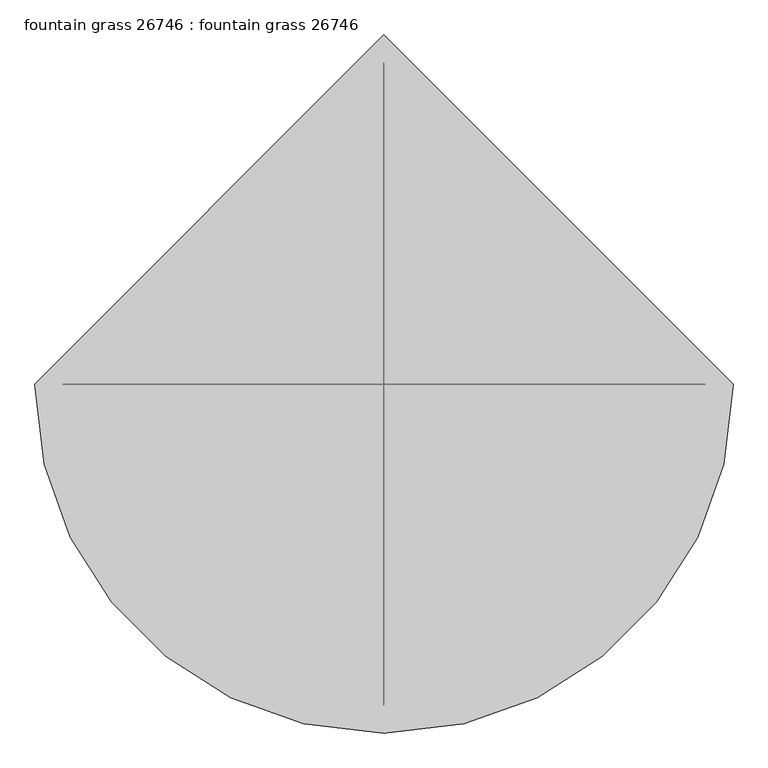
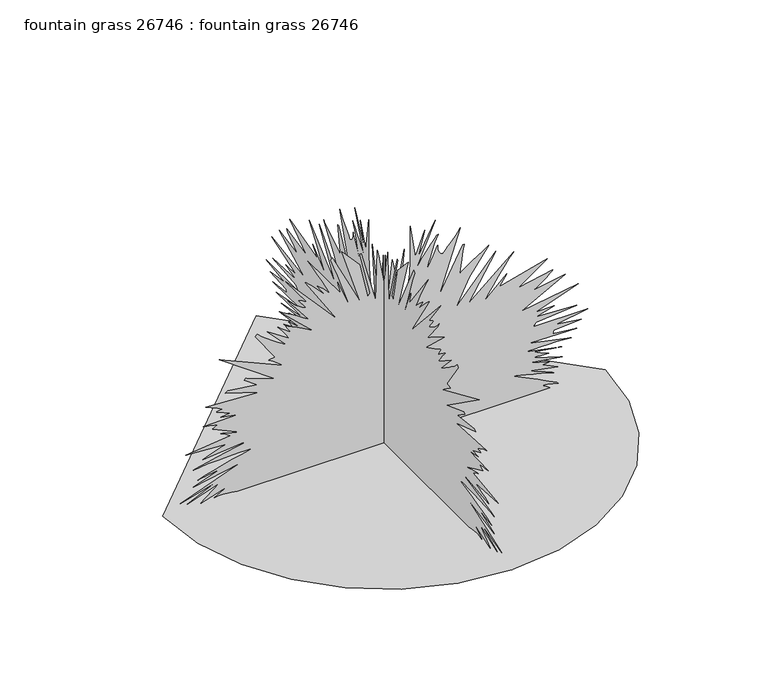
"""IFC4 building model written with IfcOpenShell, lengths in millimetres: proxy geometry, fountain grass 26746 : fountain grass 26746."""

from ifc_helpers import new_model, si_unit, origin, place, context, project, spatial, triangles, source, transform, mapped, element, save


def fountain_grass_26746_fountain_grass_26746_31a79539(model_context):
    return source(origin(), model_context, "Body", "Tessellation", [
        triangles([(-1075.1021822, 0.0, 0.0), (-1046.6796438, -246.3421583, 0.0), (-965.7324045, -472.5690837, 0.0), (-838.7452429, -672.1950891, 0.0), (-672.1950891, -838.7452429, 0.0), (-472.5690837, -965.7324045, 0.0), (-246.341904, -1046.6796438, 0.0), (4.7e-05, -1075.1021822, 0.0), (246.3421583, -1046.6796438, 0.0), (472.5690837, -965.7324045, 0.0), (672.1950891, -838.7452429, 0.0), (838.7452429, -672.1950891, 0.0), (965.7324045, -472.5690837, 0.0), (1046.6796438, -246.341904, 0.0), (1075.1021822, 9.4e-05, 0.0), (-0.000141, 1075.1021822, 0.0), (-0.0002094, 151.7493584, 903.5253731), (-0.0002064, 197.8505688, 1023.5783649), (-0.0002098, 163.2745906, 893.9190554), (-0.000206, 247.7932689, 1057.1952084), (-0.0002115, 151.7493584, 831.4910345), (-0.0002109, 167.7051159, 857.3634378), (-0.0002104, 186.8993659, 885.4837418), (-0.0002098, 207.3806375, 913.5837708), (-0.0002093, 227.1984504, 939.3926605), (-0.0002089, 244.4013429, 960.6372213), (-0.0002086, 257.0401245, 975.0516758), (-0.0002085, 263.1615169, 980.3602907), (-0.0002094, 247.7267213, 943.5176268), (-0.0002103, 234.4486256, 908.2090988), (-0.0002111, 223.4664289, 876.1391087), (-0.0002118, 214.9206206, 848.9967247), (-0.0002123, 208.9511085, 828.4836599), (-0.0002127, 205.6989088, 816.294215), (-0.0002127, 205.3039292, 814.1250887), (-0.0002127, 208.3029104, 818.0239786), (-0.0002124, 216.0537091, 832.5501995), (-0.000212, 226.6881618, 853.6500017), (-0.0002116, 238.3378685, 877.271961), (-0.0002112, 249.1338665, 899.3648712), (-0.0002109, 257.207756, 915.8748373), (-0.0002107, 260.692645, 922.748037), (-0.0002103, 260.2582965, 906.3549242), (-0.0002103, 263.0522939, 893.568568), (-0.0002106, 267.949415, 883.9953152), (-0.0002111, 273.8345936, 877.2388962), (-0.0002116, 279.5876763, 872.9031143), (-0.000212, 284.0860209, 870.5917728), (-0.0002121, 286.2119994, 869.908457), (-0.0002118, 297.8807457, 886.1644415), (-0.0002115, 309.7933362, 900.0811066), (-0.0002113, 321.8837319, 912.8293837), (-0.0002111, 334.0884012, 925.5801315), (-0.0002109, 346.3388163, 939.504427), (-0.0002105, 358.5765141, 955.7731287), (-0.0002101, 370.7304234, 975.5571682), (-0.0002182, 267.0019983, 658.6111799), (-0.000213, 382.2543929, 884.3153538), (-0.0002131, 389.9378629, 884.3153538), (-0.0002137, 385.7570498, 861.6865025), (-0.0002144, 381.2002785, 835.410272), (-0.0002152, 376.6689054, 808.0824343), (-0.0002159, 372.5719171, 782.3039932), (-0.0002165, 369.305474, 760.6733368), (-0.0002169, 367.2760194, 745.7889982), (-0.0002171, 366.8873803, 740.2492201), (-0.0002169, 377.1819918, 749.4998909), (-0.0002168, 398.429096, 764.5798571), (-0.0002166, 426.0591682, 782.8856438), (-0.0002164, 455.5053723, 801.8137035), (-0.0002163, 482.19564, 818.763105), (-0.0002161, 501.5631351, 831.122743), (-0.0002161, 509.0332824, 836.294157), (-0.0002187, 412.9883454, 706.6349201), (-0.0002218, 347.6799408, 572.1725244), (-0.0002178, 543.6077345, 793.0735394), (-0.0002226, 409.1478822, 572.1725244), (-0.0002221, 630.0006443, 760.9578398), (-0.0002225, 607.1482965, 733.4877869), (-0.0002229, 581.7076618, 698.9640947), (-0.0002232, 555.6879564, 661.3112331), (-0.0002235, 531.0982146, 624.4456781), (-0.0002238, 509.9451453, 592.2867763), (-0.000224, 494.2377829, 568.7536923), (-0.0002241, 485.9827998, 557.7656639), (-0.0002226, 597.394713, 658.6111799), (-0.0002236, 558.9747108, 605.7868607), (-0.0002249, 793.3225067, 668.217425), (-0.000226, 651.1791481, 567.3694018), (-0.0002272, 820.215996, 600.9862453), (-0.0002273, 814.2901949, 595.3652584), (-0.0002274, 803.8635057, 586.2314046), (-0.0002276, 790.0737951, 574.7607748), (-0.0002278, 774.0693214, 562.1243005), (-0.0002279, 756.9878059, 549.4928767), (-0.000228, 739.9748909, 538.045138), (-0.0002281, 724.171059, 528.951943), (-0.0002293, 881.683901, 557.7656639), (-0.0002299, 666.5461607, 442.5132874), (-0.0002323, 943.1518787, 485.7338688), (-0.0002317, 735.6975357, 413.6995302), (-0.0002329, 827.8994659, 413.6995302), (-0.0002325, 739.5380716, 389.6889682), (-0.0002353, 935.4683361, 380.0852303), (-0.0002333, 739.5380716, 360.875211), (-0.0002334, 737.0615513, 358.3860097), (-0.0002334, 734.2345436, 355.2567312), (-0.0002335, 731.3236748, 351.8201314), (-0.0002335, 728.5931728, 348.4089297), (-0.0002336, 726.3148235, 345.3558457), (-0.0002336, 724.7527096, 342.9987222), (-0.0002337, 724.171059, 341.6677714), (-0.0002372, 989.2528439, 341.6677714), (-0.0002359, 835.5829359, 317.6571731), (-0.0002381, 958.5188187, 298.4471538), (-0.0002366, 824.0564592, 288.843434), (-0.000237, 820.215996, 274.4365736), (-0.0002389, 935.4683361, 260.0296949), (-0.0002357, 704.9635832, 264.8328356), (-0.0002397, 908.5748468, 221.6119818), (-0.0002392, 879.3065025, 224.4689658), (-0.0002387, 841.8263048, 226.3310433), (-0.0002381, 800.7671831, 227.3607588), (-0.0002376, 760.7622849, 227.7214381), (-0.0002371, 726.4494083, 227.5753896), (-0.0002368, 702.461701, 227.0854304), (-0.0002367, 693.4371065, 226.4143594), (-0.0002399, 862.4738817, 192.7990239), (-0.0002375, 720.3305958, 212.0077533), (-0.0002395, 801.079664, 180.0418811), (-0.0002393, 789.8198135, 180.8544223), (-0.0002391, 775.0700598, 181.8744909), (-0.0002389, 758.976638, 182.9049694), (-0.0002386, 743.6934866, 183.7490131), (-0.0002385, 731.3642973, 184.2100133), (-0.0002384, 724.1406103, 184.090889), (-0.0002384, 724.171059, 183.194523), (-0.0002416, 866.3169611, 139.9746865), (-0.0002388, 708.8040464, 163.9857935), (-0.0002409, 802.8830423, 135.5523002), (-0.0002408, 799.4514931, 134.831959), (-0.0002408, 794.1606823, 134.0915427), (-0.0002407, 787.8817778, 133.3391994), (-0.0002407, 781.4835491, 132.5827867), (-0.0002406, 775.8346207, 131.8306978), (-0.0002406, 771.8087036, 131.0902815), (-0.0002406, 770.2720242, 130.3701946), (-0.0002426, 843.2664785, 96.75485), (-0.0002398, 697.2953739, 122.86552), (-0.0002401, 707.9455233, 119.2147799), (-0.0002406, 727.4654074, 112.0362392), (-0.0002412, 752.0246641, 102.744419), (-0.0002418, 777.7954748, 92.7543584), (-0.0002424, 800.9424631, 83.4810781), (-0.0002428, 817.6404264, 76.3393719), (-0.000243, 824.0564592, 72.7440018), (-0.0002423, 793.2310152, 81.617738), (-0.0002416, 757.9402914, 91.2158803), (-0.0002408, 721.5396063, 100.7012479), (-0.0002401, 687.3868217, 109.2361467), (-0.0002395, 658.8372562, 115.9836545), (-0.0002392, 639.2462282, 120.1060682), (-0.000239, 631.9691288, 120.7659571), (-0.00024, 666.4089598, 103.8820858), (-0.0002411, 705.799288, 84.5753155), (-0.0002422, 746.4087278, 64.5205076), (-0.0002433, 784.498554, 45.3925509), (-0.0002442, 816.3297506, 28.8660546), (-0.0002449, 838.1686792, 16.6156986), (-0.0002452, 846.2788673, 10.3164533), (-0.0002449, 834.4653442, 14.1385651), (-0.0002446, 820.7849293, 17.3725156), (-0.0002444, 806.5482256, 20.018432), (-0.0002441, 793.0684525, 22.0761847), (-0.0002439, 781.6562857, 23.5461577), (-0.0002438, 773.6197123, 24.4280193), (-0.0002437, 770.2720242, 24.7219217), (-0.0002438, 772.6468792, 22.8719915), (-0.000244, 777.9732983, 19.2397436), (-0.0002442, 785.103023, 14.5784422), (-0.0002445, 792.8881582, 9.6414491), (-0.0002447, 800.1804457, 5.1824076), (-0.0002449, 805.8319902, 1.9544036), (-0.000245, 808.6894466, 0.7109504), (-0.0002248, -712.2762182, 7.55e-05), (-0.0002247, -716.251339, 1.888295), (-0.0002245, -727.0437761, 4.4398649), (-0.0002242, -742.9644613, 7.0367071), (-0.0002239, -762.3193119, 9.0605264), (-0.0002236, -783.416498, 9.8934675), (-0.0002233, -804.5594662, 8.9170168), (-0.0002232, -824.0564592, 5.5131917), (-0.0002229, -758.7480183, 43.9307805), (-0.0002224, -893.2079069, 0.7110012), (-0.0002215, -801.0059767, 72.7440018), (-0.000221, -954.6783554, 19.9198029), (-0.000221, -820.215996, 82.3482439), (-0.0002201, -989.2528439, 34.3262887), (-0.0002208, -701.1205765, 139.9746865), (-0.0002191, -927.7848661, 96.75485), (-0.0002194, -808.6894466, 139.9746865), (-0.0002193, -812.3292681, 139.9878942), (-0.0002192, -822.1235104, 138.9035673), (-0.0002191, -836.3982931, 136.9663127), (-0.000219, -853.4747217, 134.4199656), (-0.0002188, -871.6762997, 131.5086244), (-0.0002187, -889.3216616, 128.4766238), (-0.0002185, -904.7343836, 125.5680804), (-0.0002186, -893.5940025, 129.4418265), (-0.0002187, -867.1881289, 137.4656826), (-0.0002189, -829.5479118, 148.2962261), (-0.0002191, -784.7068262, 160.5885445), (-0.0002194, -736.7034336, 172.9992332), (-0.0002196, -689.5686653, 184.1843608), (-0.0002199, -647.3361414, 192.7990239), (-0.0002198, -647.3361414, 197.6011291), (-0.0002195, -670.2748575, 197.8660475), (-0.000219, -707.9862185, 197.3700022), (-0.0002184, -755.0320387, 196.1048178), (-0.0002178, -805.9742054, 194.0624097), (-0.0002172, -855.3746058, 191.2351477), (-0.0002168, -897.79004, 187.6151289), (-0.0002165, -927.7848661, 183.194523), (-0.0002165, -918.4681383, 186.3568118), (-0.0002167, -893.3831142, 192.5249491), (-0.0002169, -856.8325836, 200.7720656), (-0.0002172, -813.1090897, 210.171837), (-0.0002176, -766.5153494, 219.7974123), (-0.0002179, -721.3516817, 228.7219402), (-0.0002182, -681.9131006, 236.0185879), (-0.0002181, -681.9131006, 240.8209655), (-0.000216, -881.683901, 221.6119818), (-0.000216, -877.2592438, 223.6533724), (-0.000216, -864.5567488, 228.9396232), (-0.000216, -846.1366522, 236.2129074), (-0.0002161, -824.5568647, 244.2159255), (-0.0002161, -802.3750065, 251.6913958), (-0.0002162, -782.1465174, 257.3830178), (-0.0002164, -766.4315609, 260.0296949), (-0.0002133, -962.3618254, 274.4365736), (-0.0002155, -747.2215416, 298.4471538), (-0.0002154, -748.9690367, 300.212453), (-0.0002152, -753.6680231, 303.7532252), (-0.000215, -760.5209478, 308.3607565), (-0.0002147, -768.7124537, 313.3315287), (-0.0002145, -777.4449875, 317.9594075), (-0.0002143, -785.9107498, 321.5357517), (-0.0002141, -793.3021591, 323.3569342), (-0.0002142, -787.9021254, 322.9682951), (-0.0002145, -773.9448378, 319.7958507), (-0.0002149, -754.7907017, 314.8758748), (-0.0002153, -733.8001951, 309.2421344), (-0.0002157, -714.3387377, 303.9360992), (-0.0002161, -699.7641912, 299.9914817), (-0.0002162, -693.4371065, 298.4471538), (-0.0002125, -831.7399292, 360.875211), (-0.0002125, -830.7239302, 362.5795401), (-0.0002124, -827.9833271, 364.8223901), (-0.0002124, -823.9904022, 367.3496704), (-0.0002124, -819.2127142, 369.9125227), (-0.0002124, -814.1174583, 372.2544219), (-0.0002124, -809.1745914, 374.1289078), (-0.0002124, -804.8489834, 375.2820714), (-0.0002124, -807.681078, 376.3869822), (-0.0002122, -815.2883898, 378.2437366), (-0.000212, -826.3196205, 380.5906863), (-0.0002117, -839.4361164, 383.168763), (-0.0002115, -853.2892679, 385.7163909), (-0.0002112, -866.5404213, 387.9770087), (-0.000211, -877.8408943, 389.6889682), (-0.0002131, -712.6470531, 394.4920907), (-0.0002116, -793.3225067, 408.8989511), (-0.0002121, -743.3810783, 413.6995302), (-0.0002103, -812.5324533, 442.5132874), (-0.0002103, -811.3640654, 443.8569191), (-0.0002103, -808.2246494, 445.132023), (-0.0002103, -803.6476032, 446.2470712), (-0.0002104, -798.178969, 447.1106812), (-0.0002104, -792.3547606, 447.6364486), (-0.0002105, -786.7133898, 447.7354978), (-0.0002106, -781.7985008, 447.31641), (-0.0002105, -785.3392731, 449.5770278), (-0.0002102, -794.7525066, 454.4588882), (-0.0002098, -808.222106, 461.0349403), (-0.0002094, -823.9294321, 468.375517), (-0.000209, -840.0584621, 475.5561107), (-0.0002086, -854.7929552, 481.6521049), (-0.0002083, -866.3169611, 485.7338688), (-0.0002122, -605.078183, 471.3270083), (-0.0002084, -770.2720242, 524.1513276), (-0.0002083, -758.7480183, 533.7550655), (-0.0002108, -616.6021889, 514.5450826), (-0.0002087, -678.0700939, 557.7656639), (-0.0002085, -670.386624, 567.3694018), (-0.0002119, -528.2407219, 514.5450826), (-0.0002026, -801.0059767, 706.6349201), (-0.0002107, -493.6662698, 572.1725244), (-0.0002103, -502.7518707, 579.84077), (-0.0002099, -513.8160936, 588.6494983), (-0.0002095, -525.7210719, 597.7502872), (-0.0002091, -537.32883, 606.3024905), (-0.0002087, -547.4989941, 613.4576134), (-0.0002085, -555.0935886, 618.3700315), (-0.0002084, -558.9772542, 620.1936848), (-0.0002084, -557.3414892, 621.3672323), (-0.0002084, -553.1149303, 622.2358566), (-0.0002085, -547.2958088, 622.8886511), (-0.0002085, -540.8924569, 623.4067881), (-0.0002086, -534.9133161, 623.8742014), (-0.0002086, -530.3616317, 624.3770777), (-0.0002086, -528.2407219, 624.99688), (-0.0002032, -624.2856588, 764.2598185), (-0.000203, -616.6021889, 773.8661362), (-0.0002039, -593.2849711, 753.716276), (-0.0002049, -567.5725871, 733.8154558), (-0.0002058, -541.6163589, 715.1616526), (-0.0002066, -517.5625946, 698.7558226), (-0.0002072, -497.5601091, 685.596088), (-0.0002077, -483.7552105, 676.68326), (-0.0002079, -478.2992935, 673.0180767), (-0.0002038, -566.6607242, 769.062941), (-0.0002074, -459.0893106, 697.0286751), (-0.0002072, -461.8096387, 701.9384771), (-0.0002069, -466.5873631, 709.5711508), (-0.0002066, -473.2904423, 719.5050648), (-0.0002061, -481.786726, 731.3211313), (-0.0002056, -491.9467163, 744.6002626), (-0.000205, -503.6332486, 758.9207548), (-0.0002044, -516.7167523, 773.8661362), (-0.0002045, -513.2318996, 772.2836746), (-0.0002048, -504.2098123, 766.0124004), (-0.0002052, -491.8044648, 756.8075117), (-0.0002057, -478.1697593, 746.4290754), (-0.0002062, -465.4570905, 736.6373766), (-0.0002065, -455.8177806, 729.1875406), (-0.0002067, -451.4058043, 725.842396), (-0.0002064, -455.2462675, 731.5675552), (-0.0002062, -459.8665524, 738.7150841), (-0.0002059, -464.8017526, 746.5230377), (-0.0002056, -469.5794769, 754.2243118), (-0.0002053, -473.7349282, 761.0594324), (-0.0002051, -476.7956062, 766.2588243), (-0.000205, -478.2992935, 769.062941), (-0.0002053, -467.4382559, 763.1752916), (-0.0002059, -448.0021966, 753.3581583), (-0.0002066, -423.3616948, 740.947724), (-0.0002073, -396.8746124, 727.2876566), (-0.0002081, -371.9089851, 713.7214788), (-0.0002087, -351.8277617, 701.5879171), (-0.0002091, -339.9964345, 692.2280233), (-0.0002022, -509.0332824, 850.7010538), (-0.0002024, -501.3497761, 846.621797), (-0.000203, -481.4362023, 834.9479456), (-0.0002039, -453.9940547, 818.4430664), (-0.0002048, -423.7299863, 799.8731243), (-0.0002057, -395.3480704, 782.0093164), (-0.0002064, -373.5523441, 767.6151369), (-0.0002068, -363.0469171, 759.4592394), (-0.0002065, -368.546, 766.7414257), (-0.0002058, -383.526917, 785.5628059), (-0.0002047, -404.1618493, 811.3869564), (-0.0002036, -426.6281379, 839.67491), (-0.0002025, -447.1030509, 865.8851561), (-0.0002018, -461.7588424, 885.4786549), (-0.0002014, -466.7727805, 893.9190554), (-0.0002023, -448.2638449, 874.4677717), (-0.000203, -430.4813184, 858.5800787), (-0.0002036, -414.1669072, 846.0858559), (-0.000204, -400.0597741, 836.8173809), (-0.0002044, -388.9066395, 830.6070768), (-0.0002046, -381.4441226, 827.2873667), (-0.0002046, -378.4138933, 826.687912), (-0.0002027, -412.9883454, 874.7116522), (-0.0002028, -410.1994168, 874.6379648), (-0.0002029, -404.7105077, 872.2808413), (-0.0002031, -397.603565, 868.4733702), (-0.0002034, -389.9581741, 864.0537998), (-0.0002036, -382.8487244, 859.8627766), (-0.0002037, -377.3623587, 856.730991), (-0.0002038, -374.5708866, 855.5016329), (-0.0001983, -478.2992935, 994.7671148), (-0.0002099, -228.5847938, 716.2386217), (-0.0002007, -382.2543929, 956.3471489), (-0.0002008, -377.5401458, 953.682704), (-0.0002013, -366.727361, 944.1653343), (-0.0002019, -351.5610629, 929.5552523), (-0.0002027, -333.7912173, 911.6203005), (-0.0002035, -315.1705153, 892.1258509), (-0.0002043, -297.4463973, 872.8294996), (-0.000205, -282.3689745, 855.5016329), (-0.0002026, -324.6294582, 917.9296537), (-0.0002027, -320.6416566, 916.0831095), (-0.000203, -312.1021706, 909.1260487), (-0.0002035, -300.8906456, 898.981319), (-0.000204, -288.8891434, 887.5817968), (-0.0002045, -277.9849398, 876.8528732), (-0.0002048, -270.0626945, 868.7172506), (-0.000205, -267.0019983, 865.1053345), (-0.0002046, -271.2920526, 874.9732641), (-0.0002037, -283.4510124, 899.7559811), (-0.0002024, -300.8601605, 934.157733), (-0.000201, -320.9083554, 972.880006), (-0.0001996, -340.9768616, 1010.6243591), (-0.0001985, -358.4571536, 1042.097438), (-0.0001977, -370.7304234, 1061.9957874), (-0.0002064, -209.3757919, 841.0947361), (-0.0002061, -212.3376932, 849.9161453), (-0.0002058, -215.4885547, 860.5994322), (-0.0002054, -218.5616956, 872.0446638), (-0.000205, -221.2901628, 883.1571396), (-0.0002047, -223.4082747, 892.8396154), (-0.0002045, -224.6477885, 899.9947746), (-0.0002044, -224.7430407, 903.5253731), (-0.0002098, -163.2748449, 749.8529943), (-0.0002094, -166.4719427, 760.9984623), (-0.0002084, -175.9733068, 790.7926466), (-0.0002069, -190.101278, 833.7744707), (-0.0002052, -207.1779428, 884.4830034), (-0.0002033, -225.5248425, 937.4622551), (-0.0002016, -243.4645905, 987.2487511), (-0.0002002, -259.318492, 1028.3814875), (-0.0002, -251.6352582, 1037.9851891), (-0.0002099, -116.1998023, 765.6542828), (-0.0002002, -205.5340569, 1052.3920858), (-0.0002042, -117.1738889, 956.3471489), (-0.00021, -78.7561757, 778.6667152), (-0.00021, -77.3934682, 780.4573763), (-0.0002099, -75.5994689, 782.9009045), (-0.0002099, -73.577631, 785.6593117), (-0.0002098, -71.5275972, 788.3949005), (-0.0002098, -69.6525708, 790.7697556), (-0.0002097, -68.1529576, 792.4410925), (-0.0002097, -67.2306846, 793.0735394), (-0.0002026, -117.1738889, 1009.1714682), (-0.0002027, -109.4901464, 1009.1714682), (-0.0002115, -40.3384626, 745.0523426), (-0.000204, -32.6549699, 999.5677666), (-0.0002043, -30.2686421, 991.1984373), (-0.0002051, -25.7212838, 968.6636209), (-0.0002061, -19.6890689, 935.823983), (-0.0002074, -12.8482471, 896.5454212), (-0.0002087, -5.8757252, 854.6837322), (-0.00021, 0.5533969, 814.1047411), (-0.0002111, 5.7626445, 778.6667152), (-0.0002057, 5.7626445, 961.1502714), (-0.0002127, 17.2877302, 730.6455185), (-0.0002072, 40.3384626, 927.5359715), (-0.0002115, 67.2306846, 793.0735394), (-0.0002069, 97.9646508, 961.1502714), (-0.0002145, 74.9141773, 697.0286751), (-0.0002143, 99.6672177, 714.3946209), (-0.0002131, 115.3773507, 759.9418407), (-0.0002114, 124.0562722, 823.853274), (-0.0002092, 127.7161506, 896.3143307), (-0.0002071, 128.3684273, 967.5027906), (-0.0002053, 128.0255249, 1027.6042093), (-0.0002042, 128.6986215, 1066.79891), (151.7493584, -7.84e-05, 903.5253731), (197.8503144, -8.55e-05, 1023.5783649), (163.2745906, -7.78e-05, 893.9190554), (247.7932689, -8.75e-05, 1057.1952084), (151.7493584, -7.41e-05, 831.4910345), (167.7048616, -7.56e-05, 857.3634378), (186.8991115, -7.73e-05, 885.4837418), (207.3803832, -7.9e-05, 913.5837708), (227.1984504, -8.05e-05, 939.3901171), (244.4013429, -8.18e-05, 960.6372213), (257.0401245, -8.26e-05, 975.0516758), (263.1615169, -8.29e-05, 980.3602907), (247.726467, -8.07e-05, 943.5176268), (234.4483712, -7.86e-05, 908.2090988), (223.4661746, -7.67e-05, 876.1391087), (214.9203662, -7.51e-05, 848.9967247), (208.9508542, -7.39e-05, 828.4811165), (205.6986544, -7.32e-05, 816.294215), (205.3036749, -7.3e-05, 814.1250887), (208.3026561, -7.32e-05, 818.0239786), (216.0534548, -7.4e-05, 832.5501995), (226.6879074, -7.52e-05, 853.6500017), (238.3376142, -7.65e-05, 877.271961), (249.1336122, -7.77e-05, 899.3623278), (257.207756, -7.86e-05, 915.8748373), (260.692645, -7.9e-05, 922.748037), (260.2582965, -7.89e-05, 906.3549242), (263.0522939, -7.86e-05, 893.568568), (267.949415, -7.8e-05, 883.9953152), (273.8345936, -7.75e-05, 877.2388962), (279.5876763, -7.69e-05, 872.9031143), (284.0860209, -7.65e-05, 870.5917728), (286.2119994, -7.64e-05, 869.908457), (297.8807457, -7.73e-05, 886.1644415), (309.7933362, -7.82e-05, 900.0811066), (321.8837319, -7.89e-05, 912.8293837), (334.0884012, -7.97e-05, 925.5801315), (346.3388163, -8.05e-05, 939.504427), (358.5765141, -8.15e-05, 955.7731287), (370.7304234, -8.27e-05, 975.5571682), (267.0019983, -6.38e-05, 658.6111799), (382.2543929, -7.72e-05, 884.3153538), (389.9378629, -7.72e-05, 884.3153538), (385.7570498, -7.59e-05, 861.6865025), (381.2002785, -7.43e-05, 835.410272), (376.6689054, -7.27e-05, 808.0824343), (372.5693736, -7.11e-05, 782.3039932), (369.305474, -6.98e-05, 760.6733368), (367.2760194, -6.9e-05, 745.7889982), (366.8873803, -6.86e-05, 740.2492201), (377.1819918, -6.92e-05, 749.4998909), (398.429096, -7.01e-05, 764.5798571), (426.0591682, -7.12e-05, 782.8856438), (455.5053723, -7.23e-05, 801.8137035), (482.19564, -7.33e-05, 818.763105), (501.5631351, -7.4e-05, 831.122743), (509.0332824, -7.43e-05, 836.294157), (412.9883454, -6.66e-05, 706.6349201), (347.6799408, -5.86e-05, 572.1725244), (543.6077345, -7.18e-05, 793.0735394), (409.1478822, -5.86e-05, 572.1725244), (629.9981009, -6.77e-05, 760.9578398), (607.145753, -6.62e-05, 733.4877869), (581.7076618, -6.44e-05, 698.9640947), (555.6879564, -6.26e-05, 661.3112331), (531.0982146, -6.09e-05, 624.4456781), (509.9451453, -5.94e-05, 592.2867763), (494.2377829, -5.83e-05, 568.7536923), (485.9827998, -5.77e-05, 557.7656639), (597.3921696, -6.38e-05, 658.6111799), (558.9747108, -6.06e-05, 605.7868607), (793.3225067, -6.43e-05, 668.217425), (651.1791481, -5.83e-05, 567.3694018), (820.215996, -6.03e-05, 600.9862453), (814.2901949, -6e-05, 595.3652584), (803.8635057, -5.94e-05, 586.2314046), (790.0737951, -5.88e-05, 574.7607748), (774.0693214, -5.8e-05, 562.1243005), (756.9878059, -5.73e-05, 549.4928767), (739.9748909, -5.66e-05, 538.045138), (724.171059, -5.6e-05, 528.951943), (881.683901, -5.77e-05, 557.7656639), (666.5461607, -5.09e-05, 442.5132874), (943.1518787, -5.35e-05, 485.7338688), (735.6975357, -4.92e-05, 413.6995302), (827.8994659, -4.92e-05, 413.6995302), (739.5380716, -4.77e-05, 389.6889682), (935.4683361, -4.72e-05, 380.0852303), (739.5380716, -4.6e-05, 360.875211), (737.0615513, -4.59e-05, 358.3860097), (734.2345436, -4.57e-05, 355.2567312), (731.3236748, -4.55e-05, 351.8201314), (728.5931728, -4.53e-05, 348.4089297), (726.3148235, -4.51e-05, 345.3558457), (724.7527096, -4.49e-05, 342.9987222), (724.171059, -4.49e-05, 341.6677714), (989.2528439, -4.49e-05, 341.6677714), (835.5829359, -4.34e-05, 317.6571731), (958.5188187, -4.23e-05, 298.4471538), (824.0564592, -4.17e-05, 288.843434), (820.215996, -4.09e-05, 274.4365736), (935.4683361, -4e-05, 260.0296949), (704.9635832, -4.03e-05, 264.8328356), (908.5748468, -3.77e-05, 221.6119818), (879.3065025, -3.79e-05, 224.4689658), (841.8263048, -3.8e-05, 226.3310433), (800.7647123, -3.81e-05, 227.3607588), (760.7622849, -3.81e-05, 227.7211837), (726.4494083, -3.81e-05, 227.5753896), (702.461701, -3.8e-05, 227.0854304), (693.4371065, -3.8e-05, 226.4141051), (862.4738817, -3.6e-05, 192.7987696), (720.3305958, -3.71e-05, 212.007499), (801.079664, -3.52e-05, 180.0418811), (789.8198135, -3.53e-05, 180.8544223), (775.0700598, -3.53e-05, 181.8744909), (758.976638, -3.54e-05, 182.9049694), (743.6934866, -3.55e-05, 183.7490131), (731.3642973, -3.55e-05, 184.2100133), (724.1406103, -3.55e-05, 184.090889), (724.171059, -3.54e-05, 183.194523), (866.3169611, -3.28e-05, 139.9746865), (708.8040464, -3.43e-05, 163.9857935), (802.8830423, -3.26e-05, 135.5523002), (799.4514931, -3.25e-05, 134.831959), (794.1606823, -3.25e-05, 134.0915427), (787.8817778, -3.24e-05, 133.3391994), (781.4810057, -3.24e-05, 132.5827867), (775.8346207, -3.24e-05, 131.8306978), (771.8087036, -3.23e-05, 131.0902815), (770.2720242, -3.23e-05, 130.3701946), (843.2664785, -3.03e-05, 96.75485), (697.2953739, -3.18e-05, 122.8652657), (707.9455233, -3.16e-05, 119.2147799), (727.4654074, -3.12e-05, 112.0362392), (752.0246641, -3.06e-05, 102.744419), (777.7954748, -3e-05, 92.7543584), (800.9424631, -2.95e-05, 83.4810781), (817.6404264, -2.91e-05, 76.3393719), (824.0564592, -2.88e-05, 72.7440018), (793.2310152, -2.94e-05, 81.617738), (757.9402914, -2.99e-05, 91.2158803), (721.5396063, -3.05e-05, 100.7012479), (687.3868217, -3.1e-05, 109.2361467), (658.8372562, -3.14e-05, 115.9836545), (639.2462282, -3.17e-05, 120.1060682), (631.9691288, -3.17e-05, 120.7659571), (666.4089598, -3.07e-05, 103.8820858), (705.799288, -2.95e-05, 84.5753155), (746.4087278, -2.83e-05, 64.5205076), (784.498554, -2.72e-05, 45.3925509), (816.3297506, -2.62e-05, 28.8660546), (838.1686792, -2.55e-05, 16.6156986), (846.2788673, -2.51e-05, 10.3164533), (834.4653442, -2.53e-05, 14.1385651), (820.7849293, -2.55e-05, 17.3724907), (806.5482256, -2.57e-05, 20.018432), (793.0684525, -2.58e-05, 22.0761598), (781.6562857, -2.59e-05, 23.5461577), (773.6197123, -2.6e-05, 24.4280193), (770.2720242, -2.6e-05, 24.7219217), (772.6468792, -2.59e-05, 22.8719915), (777.9732983, -2.56e-05, 19.2397436), (785.103023, -2.54e-05, 14.5784422), (792.8881582, -2.51e-05, 9.6414491), (800.1804457, -2.48e-05, 5.1824076), (805.8319902, -2.46e-05, 1.9544036), (808.6894466, -2.45e-05, 0.7109504), (-712.2762182, -2.45e-05, 3.05e-05), (-716.251339, -2.46e-05, 1.8882493), (-727.0437761, -2.48e-05, 4.4398141), (-742.9644613, -2.49e-05, 7.0366566), (-762.3193119, -2.5e-05, 9.0604759), (-783.416498, -2.51e-05, 9.8934175), (-804.5594662, -2.5e-05, 8.9169657), (-824.0564592, -2.48e-05, 5.5131406), (-758.7480183, -2.71e-05, 43.9307805), (-893.2104504, -2.45e-05, 0.7109504), (-801.0059767, -2.88e-05, 72.7440018), (-954.6783554, -2.57e-05, 19.919753), (-820.215996, -2.94e-05, 82.3482439), (-989.2528439, -2.65e-05, 34.3262887), (-701.1205765, -3.28e-05, 139.9746865), (-927.7848661, -3.03e-05, 96.75485), (-808.6894466, -3.28e-05, 139.9746865), (-812.3292681, -3.28e-05, 139.9878942), (-822.1235104, -3.28e-05, 138.9035673), (-836.3982931, -3.27e-05, 136.9663127), (-853.4747217, -3.25e-05, 134.4197112), (-871.6762997, -3.23e-05, 131.5086244), (-889.3216616, -3.22e-05, 128.4766238), (-904.7343836, -3.2e-05, 125.5680804), (-893.5940025, -3.22e-05, 129.4418265), (-867.1881289, -3.27e-05, 137.4656826), (-829.5479118, -3.33e-05, 148.2959718), (-784.7068262, -3.41e-05, 160.5885445), (-736.7034336, -3.48e-05, 172.9992332), (-689.5686653, -3.55e-05, 184.1841064), (-647.3361414, -3.6e-05, 192.7987696), (-647.3361414, -3.63e-05, 197.6011291), (-670.2748575, -3.63e-05, 197.8660475), (-707.9862185, -3.63e-05, 197.3700022), (-755.0320387, -3.62e-05, 196.1045634), (-805.9767488, -3.61e-05, 194.0621554), (-855.3746058, -3.59e-05, 191.2351477), (-897.79004, -3.57e-05, 187.6151289), (-927.7848661, -3.54e-05, 183.194523), (-918.4681383, -3.56e-05, 186.3568118), (-893.3831142, -3.6e-05, 192.5249491), (-856.8325836, -3.65e-05, 200.7720656), (-813.1090897, -3.7e-05, 210.1715827), (-766.5153494, -3.76e-05, 219.797158), (-721.3516817, -3.81e-05, 228.7216859), (-681.9131006, -3.86e-05, 236.0185879), (-681.9131006, -3.89e-05, 240.8207112), (-881.683901, -3.77e-05, 221.6119818), (-877.2592438, -3.78e-05, 223.6533724), (-864.5567488, -3.81e-05, 228.9396232), (-846.1391956, -3.86e-05, 236.2129074), (-824.5568647, -3.91e-05, 244.2156711), (-802.3750065, -3.95e-05, 251.6913958), (-782.1465174, -3.98e-05, 257.3804744), (-766.4315609, -4e-05, 260.0296949), (-962.3618254, -4.09e-05, 274.4365736), (-747.2215416, -4.23e-05, 298.4471538), (-748.9690367, -4.24e-05, 300.212453), (-753.6705666, -4.26e-05, 303.7532252), (-760.5209478, -4.29e-05, 308.3607565), (-768.7149971, -4.32e-05, 313.3315287), (-777.4475309, -4.35e-05, 317.9594075), (-785.9107498, -4.37e-05, 321.5357517), (-793.3021591, -4.38e-05, 323.3569342), (-787.9021254, -4.38e-05, 322.9682951), (-773.9448378, -4.36e-05, 319.7958507), (-754.7907017, -4.33e-05, 314.8758748), (-733.8001951, -4.29e-05, 309.2421344), (-714.3387377, -4.26e-05, 303.9360992), (-699.7641912, -4.24e-05, 299.9914817), (-693.4371065, -4.23e-05, 298.4471538), (-831.7399292, -4.6e-05, 360.875211), (-830.7239302, -4.61e-05, 362.5795401), (-827.9833271, -4.62e-05, 364.8223901), (-823.9929457, -4.64e-05, 367.3496704), (-819.2127142, -4.66e-05, 369.9099792), (-814.1174583, -4.67e-05, 372.2544219), (-809.1745914, -4.68e-05, 374.1289078), (-804.8489834, -4.69e-05, 375.2820714), (-807.681078, -4.69e-05, 376.3869822), (-815.2883898, -4.7e-05, 378.2437366), (-826.3196205, -4.72e-05, 380.5906863), (-839.4361164, -4.73e-05, 383.168763), (-853.2918114, -4.75e-05, 385.7163909), (-866.5404213, -4.76e-05, 387.9770087), (-877.8408943, -4.77e-05, 389.6889682), (-712.6470531, -4.8e-05, 394.4920907), (-793.3225067, -4.89e-05, 408.8989511), (-743.3810783, -4.92e-05, 413.6995302), (-812.5324533, -5.09e-05, 442.5132874), (-811.3640654, -5.1e-05, 443.8569191), (-808.2246494, -5.1e-05, 445.132023), (-803.6501467, -5.11e-05, 446.2445277), (-798.178969, -5.12e-05, 447.1106812), (-792.3547606, -5.12e-05, 447.6364486), (-786.7133898, -5.12e-05, 447.7354978), (-781.7985008, -5.12e-05, 447.31641), (-785.3392731, -5.13e-05, 449.5770278), (-794.7525066, -5.16e-05, 454.4588882), (-808.222106, -5.2e-05, 461.0349403), (-823.9294321, -5.24e-05, 468.375517), (-840.0584621, -5.28e-05, 475.5561107), (-854.7929552, -5.32e-05, 481.6521049), (-866.3169611, -5.35e-05, 485.7338688), (-605.078183, -5.26e-05, 471.3270083), (-770.2720242, -5.57e-05, 524.1513276), (-758.7480183, -5.63e-05, 533.7550655), (-616.6021889, -5.52e-05, 514.5450826), (-678.0700939, -5.77e-05, 557.7656639), (-670.386624, -5.83e-05, 567.3694018), (-528.2432653, -5.52e-05, 514.5450826), (-801.0059767, -6.66e-05, 706.6349201), (-493.6662698, -5.86e-05, 572.1725244), (-502.7518707, -5.91e-05, 579.84077), (-513.8160936, -5.96e-05, 588.6494983), (-525.7210719, -6.01e-05, 597.7502872), (-537.32883, -6.06e-05, 606.3024905), (-547.4989941, -6.11e-05, 613.4576134), (-555.0935886, -6.14e-05, 618.3700315), (-558.9772542, -6.15e-05, 620.1936848), (-557.3440327, -6.15e-05, 621.3672323), (-553.1149303, -6.16e-05, 622.2358566), (-547.2958088, -6.16e-05, 622.8886511), (-540.8924569, -6.17e-05, 623.4042446), (-534.9133161, -6.17e-05, 623.8742014), (-530.3616317, -6.17e-05, 624.3770777), (-528.2432653, -6.18e-05, 624.99688), (-624.2856588, -7.01e-05, 764.2598185), (-616.6021889, -7.06e-05, 773.8635927), (-593.2849711, -6.94e-05, 753.716276), (-567.5725871, -6.82e-05, 733.8154558), (-541.6163589, -6.71e-05, 715.1616526), (-517.5625946, -6.62e-05, 698.7558226), (-497.5601091, -6.54e-05, 685.596088), (-483.7552105, -6.48e-05, 676.68326), (-478.2992935, -6.46e-05, 673.0180767), (-566.6607242, -7.03e-05, 769.062941), (-459.091854, -6.6e-05, 697.0286751), (-461.8096387, -6.63e-05, 701.9384771), (-466.5873631, -6.68e-05, 709.5711508), (-473.2904423, -6.74e-05, 719.5050648), (-481.786726, -6.81e-05, 731.3211313), (-491.9467163, -6.89e-05, 744.6002626), (-503.6332486, -6.97e-05, 758.9207548), (-516.7167523, -7.06e-05, 773.8635927), (-513.2318996, -7.05e-05, 772.2836746), (-504.2098123, -7.02e-05, 766.0124004), (-491.8044648, -6.96e-05, 756.8075117), (-478.1697593, -6.9e-05, 746.4290754), (-465.4570905, -6.84e-05, 736.6373766), (-455.8177806, -6.8e-05, 729.1875406), (-451.4058043, -6.78e-05, 725.842396), (-455.2462675, -6.81e-05, 731.5675552), (-459.8665524, -6.85e-05, 738.7150841), (-464.8017526, -6.9e-05, 746.5230377), (-469.5794769, -6.95e-05, 754.2243118), (-473.7349282, -6.99e-05, 761.0594324), (-476.7981497, -7.02e-05, 766.2588243), (-478.2992935, -7.03e-05, 769.062941), (-467.4382559, -7e-05, 763.1752916), (-448.0021966, -6.94e-05, 753.3581583), (-423.3616948, -6.87e-05, 740.947724), (-396.8746124, -6.79e-05, 727.2876566), (-371.9089851, -6.7e-05, 713.7214788), (-351.8277617, -6.63e-05, 701.5879171), (-339.9964345, -6.58e-05, 692.2280233), (-509.0332824, -7.52e-05, 850.7010538), (-501.3497761, -7.5e-05, 846.621797), (-481.4362023, -7.43e-05, 834.9479456), (-453.9940547, -7.33e-05, 818.4430664), (-423.7299863, -7.22e-05, 799.8731243), (-395.3480704, -7.11e-05, 782.0093164), (-373.5523441, -7.03e-05, 767.6151369), (-363.0469171, -6.98e-05, 759.4592394), (-368.546, -7.02e-05, 766.7414257), (-383.526917, -7.13e-05, 785.5628059), (-404.1618493, -7.29e-05, 811.3869564), (-426.6281379, -7.46e-05, 839.67491), (-447.1030509, -7.61e-05, 865.8851561), (-461.7588424, -7.73e-05, 885.4786549), (-466.7727805, -7.78e-05, 893.9190554), (-448.2638449, -7.66e-05, 874.4677717), (-430.4813184, -7.57e-05, 858.5800787), (-414.1669072, -7.49e-05, 846.0858559), (-400.0623176, -7.44e-05, 836.8173809), (-388.9066395, -7.4e-05, 830.6070768), (-381.4441226, -7.38e-05, 827.2873667), (-378.4138933, -7.38e-05, 826.687912), (-412.9883454, -7.66e-05, 874.7116522), (-410.1994168, -7.66e-05, 874.6379648), (-404.7105077, -7.65e-05, 872.2808413), (-397.603565, -7.63e-05, 868.4733702), (-389.9581741, -7.6e-05, 864.0537998), (-382.8487244, -7.58e-05, 859.8627766), (-377.3623587, -7.56e-05, 856.730991), (-374.5708866, -7.55e-05, 855.5016329), (-478.2992935, -8.38e-05, 994.7671148), (-228.5850482, -6.72e-05, 716.2386217), (-382.2543929, -8.15e-05, 956.3471489), (-377.5401458, -8.13e-05, 953.682704), (-366.727361, -8.08e-05, 944.1653343), (-351.5610629, -7.99e-05, 929.5552523), (-333.7912173, -7.88e-05, 911.6203005), (-315.1730587, -7.77e-05, 892.1258509), (-297.4463973, -7.65e-05, 872.8294996), (-282.3689745, -7.55e-05, 855.5016329), (-324.6294582, -7.92e-05, 917.9296537), (-320.6442, -7.91e-05, 916.0831095), (-312.1021706, -7.87e-05, 909.1260487), (-300.8906456, -7.81e-05, 898.981319), (-288.8891434, -7.74e-05, 887.5817968), (-277.9874833, -7.68e-05, 876.8528732), (-270.0626945, -7.63e-05, 868.7172506), (-267.0019983, -7.61e-05, 865.1053345), (-271.2920526, -7.67e-05, 874.9732641), (-283.4510124, -7.81e-05, 899.7559811), (-300.8601605, -8.02e-05, 934.157733), (-320.9083554, -8.25e-05, 972.880006), (-340.9768616, -8.47e-05, 1010.6243591), (-358.4571536, -8.66e-05, 1042.097438), (-370.7304234, -8.78e-05, 1061.9957874), (-209.3760462, -7.46e-05, 841.0947361), (-212.3379476, -7.52e-05, 849.9161453), (-215.4885547, -7.58e-05, 860.5994322), (-218.5616956, -7.65e-05, 872.0446638), (-221.2904171, -7.71e-05, 883.1571396), (-223.4082747, -7.77e-05, 892.8396154), (-224.6480428, -7.81e-05, 899.9947746), (-224.7430407, -7.84e-05, 903.5253731), (-163.2750993, -6.92e-05, 749.8529943), (-166.4719427, -6.99e-05, 760.9984623), (-175.9735611, -7.16e-05, 790.7901031), (-190.1015323, -7.42e-05, 833.7719273), (-207.1779428, -7.72e-05, 884.4830034), (-225.5250968, -8.04e-05, 937.4622551), (-243.4648448, -8.33e-05, 987.2487511), (-259.318492, -8.58e-05, 1028.3814875), (-251.6355125, -8.64e-05, 1037.9851891), (-116.2000566, -7.01e-05, 765.6542828), (-205.5343112, -8.72e-05, 1052.3920858), (-117.1738889, -8.15e-05, 956.3471489), (-78.7564301, -7.09e-05, 778.6667152), (-77.3934682, -7.1e-05, 780.4573763), (-75.5999776, -7.12e-05, 782.9009045), (-73.5778853, -7.13e-05, 785.6593117), (-71.5278515, -7.15e-05, 788.3949005), (-69.6528251, -7.16e-05, 790.7697556), (-68.1529576, -7.17e-05, 792.4410925), (-67.2311933, -7.18e-05, 793.0735394), (-117.1738889, -8.47e-05, 1009.1714682), (-109.4904008, -8.47e-05, 1009.1714682), (-40.3384626, -6.89e-05, 745.0523426), (-32.6552242, -8.41e-05, 999.5677666), (-30.2688964, -8.36e-05, 991.1984373), (-25.7212838, -8.22e-05, 968.6636209), (-19.6892211, -8.03e-05, 935.823983), (-12.8484243, -7.79e-05, 896.5454212), (-5.8759029, -7.54e-05, 854.6837322), (0.5532267, -7.3e-05, 814.1047411), (5.7624668, -7.09e-05, 778.6667152), (5.7624668, -8.18e-05, 961.1502714), (17.2875781, -6.81e-05, 730.6455185), (40.3382082, -7.98e-05, 927.5359715), (67.2306846, -7.18e-05, 793.0735394), (97.9646508, -8.18e-05, 961.1502714), (74.9141773, -6.6e-05, 697.0286751), (99.6669633, -6.71e-05, 714.3946209), (115.3770963, -6.98e-05, 759.9418407), (124.0560179, -7.36e-05, 823.853274), (127.7158962, -7.79e-05, 896.3143307), (128.3679186, -8.22e-05, 967.5027906), (128.0250162, -8.58e-05, 1027.6042093), (128.6986215, -8.81e-05, 1066.79891)], [[15, 16, 1], [14, 15, 1], [14, 1, 2], [13, 14, 2], [13, 2, 3], [13, 3, 4], [12, 13, 4], [11, 12, 4], [11, 4, 5], [11, 5, 6], [11, 6, 7], [11, 7, 8], [11, 8, 9], [11, 9, 10], [127, 128, 129], [197, 198, 199], [444, 445, 446], [117, 118, 119], [404, 405, 406], [19, 20, 21], [195, 196, 197], [119, 120, 121], [380, 381, 382], [448, 449, 450], [137, 138, 139], [103, 104, 105], [207, 208, 209], [112, 113, 114], [17, 18, 19], [199, 200, 201], [247, 248, 249], [403, 404, 406], [119, 121, 122], [269, 270, 271], [99, 100, 101], [222, 223, 224], [222, 224, 225], [239, 240, 241], [77, 78, 79], [268, 269, 271], [295, 296, 297], [114, 115, 116], [402, 403, 406], [75, 76, 77], [155, 156, 157], [154, 155, 157], [267, 268, 271], [456, 457, 17], [119, 122, 123], [85, 86, 87], [147, 148, 149], [101, 102, 103], [271, 272, 273], [320, 321, 322], [266, 267, 271], [455, 456, 17], [287, 288, 289], [364, 365, 366], [401, 402, 406], [363, 364, 366], [350, 351, 352], [350, 352, 353], [350, 353, 354], [77, 79, 80], [129, 130, 131], [97, 98, 99], [265, 266, 271], [55, 56, 57], [350, 354, 355], [231, 232, 233], [231, 233, 234], [231, 234, 235], [231, 235, 236], [231, 236, 237], [286, 287, 289], [129, 131, 132], [231, 237, 238], [231, 238, 239], [119, 123, 124], [191, 192, 193], [169, 170, 171], [87, 88, 89], [193, 194, 195], [72, 73, 74], [264, 265, 271], [400, 401, 406], [77, 80, 81], [285, 286, 289], [350, 355, 356], [183, 184, 185], [247, 249, 250], [246, 247, 250], [129, 132, 133], [284, 285, 289], [71, 72, 74], [436, 437, 438], [436, 438, 439], [436, 439, 440], [436, 440, 441], [54, 55, 57], [446, 447, 448], [328, 329, 330], [328, 330, 331], [139, 140, 141], [139, 141, 142], [139, 142, 143], [139, 143, 144], [283, 284, 289], [207, 209, 210], [206, 207, 210], [77, 81, 82], [350, 356, 357], [436, 441, 442], [182, 183, 185], [412, 413, 414], [411, 412, 414], [410, 411, 414], [409, 410, 414], [408, 409, 414], [407, 408, 414], [406, 407, 414], [139, 144, 145], [454, 455, 17], [70, 71, 74], [263, 264, 271], [399, 400, 406], [181, 182, 185], [282, 283, 289], [382, 383, 384], [382, 384, 385], [382, 385, 386], [382, 386, 387], [382, 387, 388], [382, 388, 389], [382, 389, 390], [180, 181, 185], [27, 28, 29], [26, 27, 29], [423, 424, 425], [423, 425, 426], [179, 180, 185], [89, 90, 91], [89, 91, 92], [89, 92, 93], [119, 124, 125], [53, 54, 57], [129, 133, 134], [153, 154, 157], [153, 157, 158], [152, 153, 158], [350, 357, 358], [178, 179, 185], [190, 191, 193], [139, 145, 146], [390, 391, 392], [390, 392, 393], [390, 393, 394], [390, 394, 395], [89, 93, 94], [41, 42, 43], [77, 82, 83], [89, 94, 95], [281, 282, 289], [177, 178, 185], [436, 442, 443], [52, 53, 57], [342, 343, 344], [69, 70, 74], [51, 52, 57], [50, 51, 57], [49, 50, 57], [89, 95, 96], [390, 395, 396], [221, 222, 225], [221, 225, 226], [398, 399, 406], [341, 342, 344], [205, 206, 210], [205, 210, 211], [204, 205, 211], [89, 96, 97], [77, 83, 84], [129, 134, 135], [195, 197, 199], [139, 146, 147], [139, 147, 149], [363, 366, 367], [362, 363, 367], [362, 367, 368], [152, 158, 159], [151, 152, 159], [245, 246, 250], [245, 250, 251], [244, 245, 251], [203, 204, 211], [372, 373, 374], [372, 374, 375], [372, 375, 376], [372, 376, 377], [372, 377, 378], [436, 443, 444], [289, 290, 291], [289, 291, 292], [77, 84, 85], [189, 190, 193], [68, 69, 74], [303, 304, 305], [446, 448, 450], [168, 169, 171], [168, 171, 172], [40, 41, 43], [328, 331, 332], [327, 328, 332], [119, 125, 126], [168, 172, 173], [372, 378, 379], [303, 305, 306], [193, 195, 199], [203, 211, 212], [202, 203, 212], [201, 202, 212], [199, 201, 212], [199, 212, 213], [199, 213, 214], [167, 168, 173], [167, 173, 174], [25, 26, 29], [25, 29, 30], [167, 174, 175], [327, 332, 333], [326, 327, 333], [24, 25, 30], [273, 274, 275], [273, 275, 276], [273, 276, 277], [273, 277, 278], [273, 278, 279], [273, 279, 280], [273, 280, 281], [273, 281, 289], [271, 273, 289], [129, 135, 136], [390, 396, 397], [361, 362, 368], [361, 368, 369], [340, 341, 344], [231, 239, 241], [243, 244, 251], [243, 251, 252], [242, 243, 252], [241, 242, 252], [231, 241, 252], [231, 252, 253], [231, 253, 254], [231, 254, 255], [89, 97, 99], [372, 379, 380], [372, 380, 382], [255, 256, 257], [255, 257, 258], [255, 258, 259], [255, 259, 260], [255, 260, 261], [255, 261, 262], [255, 262, 263], [255, 263, 271], [112, 114, 116], [150, 151, 159], [150, 159, 160], [149, 150, 160], [433, 434, 435], [433, 435, 436], [292, 293, 294], [292, 294, 295], [289, 292, 295], [326, 333, 334], [325, 326, 334], [24, 30, 31], [23, 24, 31], [436, 444, 446], [421, 422, 423], [420, 421, 423], [419, 420, 423], [418, 419, 423], [417, 418, 423], [416, 417, 423], [415, 416, 423], [414, 415, 423], [58, 59, 60], [57, 58, 60], [57, 60, 61], [57, 61, 62], [57, 62, 63], [57, 63, 64], [57, 64, 65], [57, 65, 66], [361, 369, 370], [67, 68, 74], [40, 43, 44], [23, 31, 32], [22, 23, 32], [22, 32, 33], [340, 344, 345], [339, 340, 345], [338, 339, 345], [302, 303, 306], [302, 306, 307], [188, 189, 193], [325, 334, 335], [324, 325, 335], [221, 226, 227], [220, 221, 227], [220, 227, 228], [219, 220, 228], [219, 228, 229], [218, 219, 229], [218, 229, 230], [217, 218, 230], [360, 361, 370], [360, 370, 371], [360, 371, 372], [360, 372, 382], [359, 360, 382], [358, 359, 382], [350, 358, 382], [324, 335, 336], [323, 324, 336], [167, 175, 176], [166, 167, 176], [166, 176, 177], [166, 177, 185], [165, 166, 185], [164, 165, 185], [163, 164, 185], [311, 312, 313], [311, 313, 314], [311, 314, 315], [311, 315, 316], [311, 316, 317], [311, 317, 318], [112, 116, 117], [112, 117, 119], [311, 318, 319], [302, 307, 308], [301, 302, 308], [301, 308, 309], [337, 338, 345], [337, 345, 346], [336, 337, 346], [390, 397, 398], [382, 390, 398], [382, 398, 406], [382, 406, 414], [432, 433, 436], [431, 432, 436], [430, 431, 436], [429, 430, 436], [428, 429, 436], [427, 428, 436], [426, 427, 436], [48, 49, 57], [119, 126, 127], [21, 22, 33], [21, 33, 34], [21, 34, 35], [66, 67, 74], [66, 74, 75], [57, 66, 75], [39, 40, 44], [39, 44, 45], [301, 309, 310], [300, 301, 310], [300, 310, 311], [255, 271, 289], [47, 48, 57], [453, 454, 17], [453, 17, 19], [453, 19, 21], [311, 319, 320], [216, 217, 230], [452, 453, 21], [452, 21, 35], [188, 193, 199], [187, 188, 199], [186, 187, 199], [185, 186, 199], [163, 185, 199], [163, 199, 214], [163, 214, 215], [163, 215, 216], [322, 323, 336], [46, 47, 57], [87, 89, 99], [85, 87, 99], [99, 101, 103], [99, 103, 105], [99, 105, 106], [99, 106, 107], [99, 107, 108], [99, 108, 109], [99, 109, 110], [99, 110, 111], [99, 111, 112], [300, 311, 320], [299, 300, 320], [298, 299, 320], [297, 298, 320], [149, 160, 161], [139, 149, 161], [127, 129, 136], [99, 112, 119], [39, 45, 46], [39, 46, 57], [38, 39, 57], [37, 38, 57], [36, 37, 57], [35, 36, 57], [452, 35, 57], [451, 452, 57], [423, 426, 436], [216, 230, 231], [322, 336, 346], [322, 346, 347], [85, 99, 119], [85, 119, 127], [136, 137, 139], [127, 136, 139], [127, 139, 161], [127, 161, 162], [85, 127, 162], [85, 162, 163], [85, 163, 216], [77, 85, 216], [75, 77, 216], [57, 75, 216], [57, 216, 231], [57, 231, 255], [57, 255, 289], [57, 289, 295], [57, 295, 297], [57, 297, 320], [57, 320, 322], [322, 347, 348], [450, 451, 57], [322, 348, 349], [322, 349, 350], [57, 322, 350], [450, 57, 350], [450, 350, 382], [446, 450, 382], [436, 446, 382], [436, 382, 414], [423, 436, 414], [568, 569, 570], [638, 639, 640], [885, 886, 887], [558, 559, 560], [845, 846, 847], [460, 461, 462], [636, 637, 638], [560, 561, 562], [821, 822, 823], [889, 890, 891], [578, 579, 580], [544, 545, 546], [648, 649, 650], [553, 554, 555], [458, 459, 460], [640, 641, 642], [688, 689, 690], [844, 845, 847], [560, 562, 563], [710, 711, 712], [540, 541, 542], [663, 664, 665], [663, 665, 666], [680, 681, 682], [518, 519, 520], [709, 710, 712], [736, 737, 738], [555, 556, 557], [843, 844, 847], [516, 517, 518], [596, 597, 598], [595, 596, 598], [708, 709, 712], [897, 898, 458], [560, 563, 564], [526, 527, 528], [588, 589, 590], [542, 543, 544], [712, 713, 714], [761, 762, 763], [707, 708, 712], [896, 897, 458], [728, 729, 730], [805, 806, 807], [842, 843, 847], [804, 805, 807], [791, 792, 793], [791, 793, 794], [791, 794, 795], [518, 520, 521], [570, 571, 572], [538, 539, 540], [706, 707, 712], [496, 497, 498], [791, 795, 796], [672, 673, 674], [672, 674, 675], [672, 675, 676], [672, 676, 677], [672, 677, 678], [727, 728, 730], [570, 572, 573], [672, 678, 679], [672, 679, 680], [560, 564, 565], [632, 633, 634], [610, 611, 612], [528, 529, 530], [634, 635, 636], [513, 514, 515], [705, 706, 712], [841, 842, 847], [518, 521, 522], [726, 727, 730], [791, 796, 797], [624, 625, 626], [688, 690, 691], [687, 688, 691], [570, 573, 574], [725, 726, 730], [512, 513, 515], [877, 878, 879], [877, 879, 880], [877, 880, 881], [877, 881, 882], [495, 496, 498], [887, 888, 889], [769, 770, 771], [769, 771, 772], [580, 581, 582], [580, 582, 583], [580, 583, 584], [580, 584, 585], [724, 725, 730], [648, 650, 651], [647, 648, 651], [518, 522, 523], [791, 797, 798], [877, 882, 883], [623, 624, 626], [853, 854, 855], [852, 853, 855], [851, 852, 855], [850, 851, 855], [849, 850, 855], [848, 849, 855], [847, 848, 855], [580, 585, 586], [895, 896, 458], [511, 512, 515], [704, 705, 712], [840, 841, 847], [622, 623, 626], [723, 724, 730], [823, 824, 825], [823, 825, 826], [823, 826, 827], [823, 827, 828], [823, 828, 829], [823, 829, 830], [823, 830, 831], [621, 622, 626], [468, 469, 470], [467, 468, 470], [864, 865, 866], [864, 866, 867], [620, 621, 626], [530, 531, 532], [530, 532, 533], [530, 533, 534], [560, 565, 566], [494, 495, 498], [570, 574, 575], [594, 595, 598], [594, 598, 599], [593, 594, 599], [791, 798, 799], [619, 620, 626], [631, 632, 634], [580, 586, 587], [831, 832, 833], [831, 833, 834], [831, 834, 835], [831, 835, 836], [530, 534, 535], [482, 483, 484], [518, 523, 524], [530, 535, 536], [722, 723, 730], [618, 619, 626], [877, 883, 884], [493, 494, 498], [783, 784, 785], [510, 511, 515], [492, 493, 498], [491, 492, 498], [490, 491, 498], [530, 536, 537], [831, 836, 837], [662, 663, 666], [662, 666, 667], [839, 840, 847], [782, 783, 785], [646, 647, 651], [646, 651, 652], [645, 646, 652], [530, 537, 538], [518, 524, 525], [570, 575, 576], [636, 638, 640], [580, 587, 588], [580, 588, 590], [804, 807, 808], [803, 804, 808], [803, 808, 809], [593, 599, 600], [592, 593, 600], [686, 687, 691], [686, 691, 692], [685, 686, 692], [644, 645, 652], [813, 814, 815], [813, 815, 816], [813, 816, 817], [813, 817, 818], [813, 818, 819], [877, 884, 885], [730, 731, 732], [730, 732, 733], [518, 525, 526], [630, 631, 634], [509, 510, 515], [744, 745, 746], [887, 889, 891], [609, 610, 612], [609, 612, 613], [481, 482, 484], [769, 772, 773], [768, 769, 773], [560, 566, 567], [609, 613, 614], [813, 819, 820], [744, 746, 747], [634, 636, 640], [644, 652, 653], [643, 644, 653], [642, 643, 653], [640, 642, 653], [640, 653, 654], [640, 654, 655], [608, 609, 614], [608, 614, 615], [466, 467, 470], [466, 470, 471], [608, 615, 616], [768, 773, 774], [767, 768, 774], [465, 466, 471], [714, 715, 716], [714, 716, 717], [714, 717, 718], [714, 718, 719], [714, 719, 720], [714, 720, 721], [714, 721, 722], [714, 722, 730], [712, 714, 730], [570, 576, 577], [831, 837, 838], [802, 803, 809], [802, 809, 810], [781, 782, 785], [672, 680, 682], [684, 685, 692], [684, 692, 693], [683, 684, 693], [682, 683, 693], [672, 682, 693], [672, 693, 694], [672, 694, 695], [672, 695, 696], [530, 538, 540], [813, 820, 821], [813, 821, 823], [696, 697, 698], [696, 698, 699], [696, 699, 700], [696, 700, 701], [696, 701, 702], [696, 702, 703], [696, 703, 704], [696, 704, 712], [553, 555, 557], [591, 592, 600], [591, 600, 601], [590, 591, 601], [874, 875, 876], [874, 876, 877], [733, 734, 735], [733, 735, 736], [730, 733, 736], [767, 774, 775], [766, 767, 775], [465, 471, 472], [464, 465, 472], [877, 885, 887], [862, 863, 864], [861, 862, 864], [860, 861, 864], [859, 860, 864], [858, 859, 864], [857, 858, 864], [856, 857, 864], [855, 856, 864], [499, 500, 501], [498, 499, 501], [498, 501, 502], [498, 502, 503], [498, 503, 504], [498, 504, 505], [498, 505, 506], [498, 506, 507], [802, 810, 811], [508, 509, 515], [481, 484, 485], [464, 472, 473], [463, 464, 473], [463, 473, 474], [781, 785, 786], [780, 781, 786], [779, 780, 786], [743, 744, 747], [743, 747, 748], [629, 630, 634], [766, 775, 776], [765, 766, 776], [662, 667, 668], [661, 662, 668], [661, 668, 669], [660, 661, 669], [660, 669, 670], [659, 660, 670], [659, 670, 671], [658, 659, 671], [801, 802, 811], [801, 811, 812], [801, 812, 813], [801, 813, 823], [800, 801, 823], [799, 800, 823], [791, 799, 823], [765, 776, 777], [764, 765, 777], [608, 616, 617], [607, 608, 617], [607, 617, 618], [607, 618, 626], [606, 607, 626], [605, 606, 626], [604, 605, 626], [752, 753, 754], [752, 754, 755], [752, 755, 756], [752, 756, 757], [752, 757, 758], [752, 758, 759], [553, 557, 558], [553, 558, 560], [752, 759, 760], [743, 748, 749], [742, 743, 749], [742, 749, 750], [778, 779, 786], [778, 786, 787], [777, 778, 787], [831, 838, 839], [823, 831, 839], [823, 839, 847], [823, 847, 855], [873, 874, 877], [872, 873, 877], [871, 872, 877], [870, 871, 877], [869, 870, 877], [868, 869, 877], [867, 868, 877], [489, 490, 498], [560, 567, 568], [462, 463, 474], [462, 474, 475], [462, 475, 476], [507, 508, 515], [507, 515, 516], [498, 507, 516], [480, 481, 485], [480, 485, 486], [742, 750, 751], [741, 742, 751], [741, 751, 752], [696, 712, 730], [488, 489, 498], [894, 895, 458], [894, 458, 460], [894, 460, 462], [752, 760, 761], [657, 658, 671], [893, 894, 462], [893, 462, 476], [629, 634, 640], [628, 629, 640], [627, 628, 640], [626, 627, 640], [604, 626, 640], [604, 640, 655], [604, 655, 656], [604, 656, 657], [763, 764, 777], [487, 488, 498], [528, 530, 540], [526, 528, 540], [540, 542, 544], [540, 544, 546], [540, 546, 547], [540, 547, 548], [540, 548, 549], [540, 549, 550], [540, 550, 551], [540, 551, 552], [540, 552, 553], [741, 752, 761], [740, 741, 761], [739, 740, 761], [738, 739, 761], [590, 601, 602], [580, 590, 602], [568, 570, 577], [540, 553, 560], [480, 486, 487], [480, 487, 498], [479, 480, 498], [478, 479, 498], [477, 478, 498], [476, 477, 498], [893, 476, 498], [892, 893, 498], [864, 867, 877], [657, 671, 672], [763, 777, 787], [763, 787, 788], [526, 540, 560], [526, 560, 568], [577, 578, 580], [568, 577, 580], [568, 580, 602], [568, 602, 603], [526, 568, 603], [526, 603, 604], [526, 604, 657], [518, 526, 657], [516, 518, 657], [498, 516, 657], [498, 657, 672], [498, 672, 696], [498, 696, 730], [498, 730, 736], [498, 736, 738], [498, 738, 761], [498, 761, 763], [763, 788, 789], [891, 892, 498], [763, 789, 790], [763, 790, 791], [498, 763, 791], [891, 498, 791], [891, 791, 823], [887, 891, 823], [877, 887, 823], [877, 823, 855], [864, 877, 855]], closed=False),
    ])


if __name__ == "__main__":
    model = new_model("IFC4")
    model_context = context("Model", 3, world=origin())
    ifc_project = project(units=[si_unit("LENGTHUNIT", "METRE", prefix="MILLI")], contexts=[model_context])
    site = spatial("IfcSite", under=ifc_project)
    building = spatial("IfcBuilding", under=site)
    placement = place(None, origin())
    fountain_grass_26746_fountain_grass_26746_shape = fountain_grass_26746_fountain_grass_26746_31a79539(model_context)
    element("IfcBuildingElementProxy", 1, Name="fountain grass 26746 : fountain grass 26746", ObjectType="fountain grass 26746 : fountain grass 26746", at=placement, inside=building, context=model_context, shape_type="MappedRepresentation", body=[
        mapped(fountain_grass_26746_fountain_grass_26746_shape, transform((0.0, 0.0, 0.0), x_axis=(1.0, 0.0, 0.0), y_axis=(0.0, 1.0, 0.0), z_axis=(0.0, 0.0, 1.0))),
    ])
    save(model, "model.ifc")

# Revit data of these elements
# Type "fountain grass 26746 : fountain grass 26746"
#   built-in parameter 1005195 = "RPC-16-G1GP-21FX-7KGL-L000-ST1L-LVER-AU"
#   Height = 0
